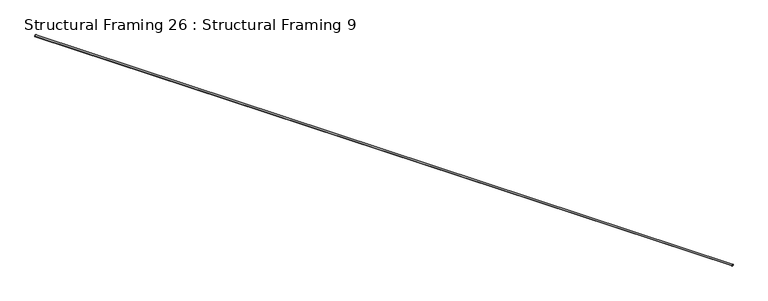
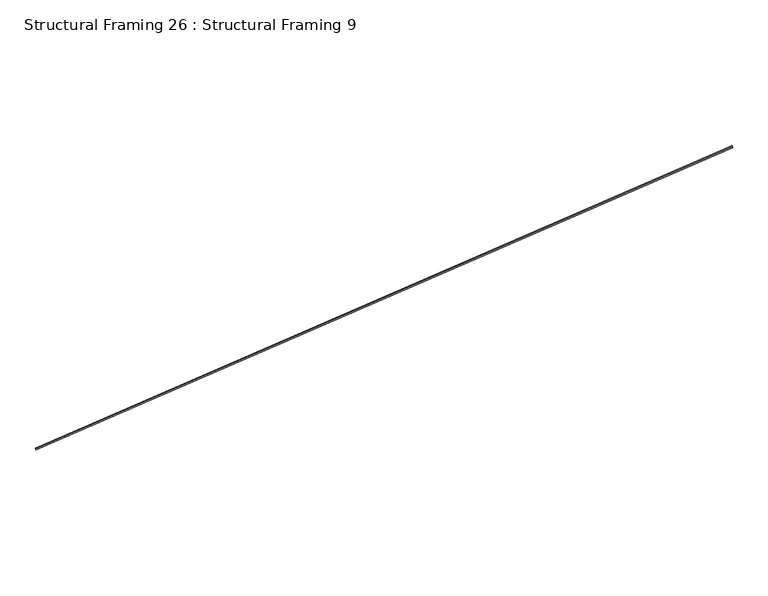
"""IFC4 building model written with IfcOpenShell, lengths in millimetres: beam geometry, Structural Framing 26 : Structural Framing 9."""

from ifc_helpers import new_model, si_unit, point, frame, origin, origin_2d, place, context, project, spatial, circle_curve, trimmed, segment, composite_curve, outline, extrude, source, transform, mapped, element, save


def structural_framing_26_structural_framing_9_6b3c6b22(model_context):
    return source(origin(), model_context, "Body", "SweptSolid", [
        extrude(outline(composite_curve([segment(trimmed(circle_curve(origin_2d(), 6.35), [point((0.0, 6.35))], [point((0.0, -6.3499999))], False, "CARTESIAN"), True, "CONTINUOUS"), segment(trimmed(circle_curve(origin_2d(), 6.35), [point((0.0, -6.3499999))], [point((0.0, 6.35))], False, "CARTESIAN"), True, "CONTINUOUS")], self_intersect=False)), frame((23270.2350052, 11682.7351788, 2966.1078019), z_axis=(0.8890536510975645, -0.29307835176728175, 0.35169402212074025), x_axis=(0.0, -0.7682212795973776, -0.6401843996644778)), (0.0, 0.0, 1.0), 5574.8064179),
    ])


if __name__ == "__main__":
    model = new_model("IFC4")
    model_context = context("Model", 3, world=origin())
    ifc_project = project(units=[si_unit("LENGTHUNIT", "METRE", prefix="MILLI")], contexts=[model_context])
    site = spatial("IfcSite", under=ifc_project)
    building = spatial("IfcBuilding", under=site)
    placement = place(None, origin())
    structural_framing_26_structural_framing_9_shape = structural_framing_26_structural_framing_9_6b3c6b22(model_context)
    element("IfcBeam", 1, ObjectType="Structural Framing 26 : Structural Framing 9", at=placement, inside=building, context=model_context, shape_type="MappedRepresentation", body=[
        mapped(structural_framing_26_structural_framing_9_shape, transform((0.0, 0.0, 0.0), x_axis=(1.0, 0.0, 0.0), y_axis=(0.0, 1.0, 0.0), z_axis=(0.0, 0.0, 1.0))),
    ])
    save(model, "model.ifc")

# Revit data of these elements
# Type "Structural Framing 26 : Structural Framing 9"
#   Structural Material [instance default] = EXISTING LATERAL BRACING (1/4" CABLE)
# Element 1 (IfcBeam, "Structural Framing 26 : Structural Framing 9")
#   Materials on its faces: "EXISTING LATERAL BRACING (1/4\" CABLE)"
# Materials
#   "EXISTING LATERAL BRACING (1/4\" CABLE)": class "Generic", colour RGB 120 120 120, transparency 0, Cost = 0
